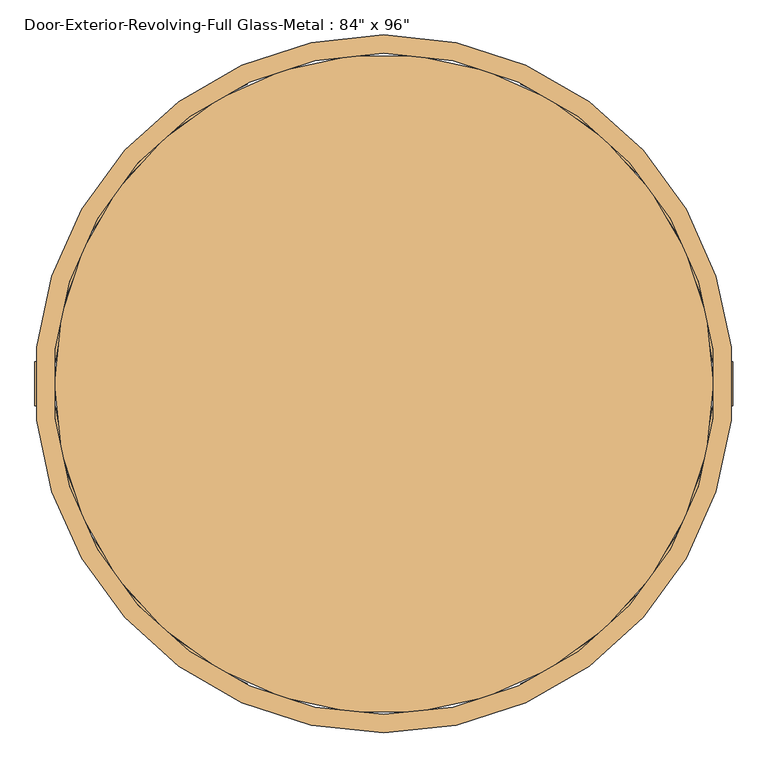
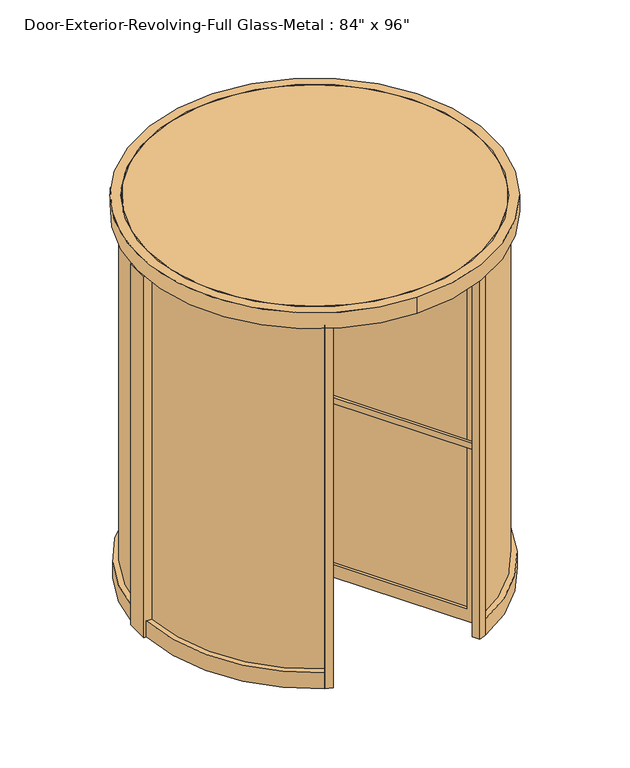
"""IFC4 building model written with IfcOpenShell, lengths in millimetres: door geometry."""

import ifcopenshell
import ifcopenshell.guid

model = None  # the IFC model being written
_history = None  # IfcOwnerHistory: only IFC2X3 demands one
_inside = {}  # id of a spatial element -> (the spatial element, [elements in it])
_under = {}  # id of a project, library or spatial element -> (it, [spatial elements below it])
_declared = {}  # id of a project -> (the project, [libraries it declares])
_typed = {}  # id of a type object -> (the type object, [elements of that type])
_made_of = {}  # id of a material, layer set ... -> (it, [elements and type objects made of it])


def new_model(schema):
    """Start an empty IFC model of exactly this schema.

    Asked for "IFC4X3", IfcOpenShell would pick the latest addendum, in which some entities
    have other attributes; the version numbers below select the first issue.
    IFC2X3 requires an IfcOwnerHistory on every rooted entity: one is made here for all.
    """
    global model, _history
    if schema == "IFC4X3":
        model = ifcopenshell.file(schema_version=(4, 3, 0, 0))
    else:
        model = ifcopenshell.file(schema=schema)
    _inside.clear()
    _under.clear()
    _declared.clear()
    _typed.clear()
    _made_of.clear()
    _history = None
    if model.schema == "IFC2X3":
        org = make("IfcOrganization", Name="unknown")
        user = make(
            "IfcPersonAndOrganization",
            ThePerson=make("IfcPerson", FamilyName="unknown"),
            TheOrganization=org,
        )
        app = make(
            "IfcApplication",
            ApplicationDeveloper=org,
            Version="unknown",
            ApplicationFullName="unknown",
            ApplicationIdentifier="unknown",
        )
        _history = make(
            "IfcOwnerHistory",
            OwningUser=user,
            OwningApplication=app,
            ChangeAction="ADDED",
            CreationDate=0,
        )
    return model


def make(cls, **values):
    """One entity of the class cls with the attributes given. An attribute that is None is left unset."""
    return model.create_entity(
        cls, **{name: value for name, value in values.items() if value is not None}
    )


def rooted(cls, **values):
    """An entity with a GlobalId (a new one), such as an element, a storey or a relation."""
    return make(cls, GlobalId=ifcopenshell.guid.new(), OwnerHistory=_history, **values)


def si_unit(unit_type, name, prefix=None):
    """IfcSIUnit, for example si_unit("LENGTHUNIT", "METRE", prefix="MILLI")."""
    return make("IfcSIUnit", UnitType=unit_type, Prefix=prefix, Name=name)


def assignment(units):
    """IfcUnitAssignment: the units of a project."""
    return None if units is None else make("IfcUnitAssignment", Units=units)


def point(xyz):
    """IfcCartesianPoint."""
    return None if xyz is None else make("IfcCartesianPoint", Coordinates=xyz)


def direction(xyz):
    """IfcDirection."""
    return None if xyz is None else make("IfcDirection", DirectionRatios=xyz)


def frame(location, z_axis=None, x_axis=None):
    """IfcAxis2Placement3D, a coordinate frame: its origin and axes. An axis left out is left unset."""
    return make(
        "IfcAxis2Placement3D",
        Location=point(location),
        Axis=direction(z_axis),
        RefDirection=direction(x_axis),
    )


def frame_2d(location, x_axis=None):
    """IfcAxis2Placement2D, a coordinate frame in the plane: its origin and x axis."""
    return make(
        "IfcAxis2Placement2D", Location=point(location), RefDirection=direction(x_axis)
    )


def origin():
    """The frame at (0, 0, 0) with its axes left unset."""
    return frame((0.0, 0.0, 0.0))


def origin_with_axes():
    """The frame at (0, 0, 0) with the z axis (0, 0, 1) and the x axis (1, 0, 0) written out."""
    return frame((0.0, 0.0, 0.0), z_axis=(0.0, 0.0, 1.0), x_axis=(1.0, 0.0, 0.0))


def origin_2d():
    """The frame at (0, 0) in the plane with its x axis left unset."""
    return frame_2d((0.0, 0.0))


def place(relative_to, where):
    """IfcLocalPlacement: puts the frame where relative to a parent placement (None: the world)."""
    return make(
        "IfcLocalPlacement", PlacementRelTo=relative_to, RelativePlacement=where
    )


def context(
    kind, dimensions, precision=None, world=None, true_north=None, identifier=None
):
    """IfcGeometricRepresentationContext, for example the 3D "Model" context."""
    return make(
        "IfcGeometricRepresentationContext",
        ContextIdentifier=identifier,
        ContextType=kind,
        CoordinateSpaceDimension=dimensions,
        Precision=precision,
        WorldCoordinateSystem=world,
        TrueNorth=true_north,
    )


def project(units=None, contexts=None):
    """IfcProject with its units and contexts."""
    return rooted(
        "IfcProject",
        Name="project",
        RepresentationContexts=contexts,
        UnitsInContext=assignment(units),
    )


def spatial(cls, under=None, at=None, **own):
    """A site, building, storey or space (cls), placed at a placement, below another one or the project."""
    s = rooted(cls, ObjectPlacement=at, **own)
    if under is not None:
        _under.setdefault(under.id(), (under, []))[1].append(s)
    return s


def polyline(points):
    """IfcPolyline through the points."""
    return make("IfcPolyline", Points=[point(p) for p in points])


def circle_curve(where, radius):
    """IfcCircle in the frame where."""
    return make("IfcCircle", Position=where, Radius=radius)


def trimmed(basis, trim1, trim2, sense, master):
    """IfcTrimmedCurve: the piece of a basis curve between two trims."""
    return make(
        "IfcTrimmedCurve",
        BasisCurve=basis,
        Trim1=trim1,
        Trim2=trim2,
        SenseAgreement=sense,
        MasterRepresentation=master,
    )


def segment(curve, same_sense, transition):
    """IfcCompositeCurveSegment."""
    return make(
        "IfcCompositeCurveSegment",
        Transition=transition,
        SameSense=same_sense,
        ParentCurve=curve,
    )


def composite_curve(segments, self_intersect=None):
    """IfcCompositeCurve: segments joined end to end."""
    return make("IfcCompositeCurve", Segments=segments, SelfIntersect=self_intersect)


def outline(outer, holes=None, kind="AREA"):
    """IfcArbitraryClosedProfileDef: a profile drawn as a closed curve; with holes, ...WithVoids."""
    if holes is None:
        return make("IfcArbitraryClosedProfileDef", ProfileType=kind, OuterCurve=outer)
    return make(
        "IfcArbitraryProfileDefWithVoids",
        ProfileType=kind,
        OuterCurve=outer,
        InnerCurves=holes,
    )


def extrude(swept, where, along, depth):
    """IfcExtrudedAreaSolid: the profile swept, set in the frame where, extruded along a direction by depth."""
    return make(
        "IfcExtrudedAreaSolid",
        SweptArea=swept,
        Position=where,
        ExtrudedDirection=direction(along),
        Depth=depth,
    )


def shape(context_of_items, identifier, shape_type, items):
    """IfcShapeRepresentation: the items that make up one representation, for example the "Body"."""
    return make(
        "IfcShapeRepresentation",
        ContextOfItems=context_of_items,
        RepresentationIdentifier=identifier,
        RepresentationType=shape_type,
        Items=items,
    )


def source(mapping_origin, context_of_items, identifier, shape_type, items):
    """IfcRepresentationMap: a shape defined once, which mapped items show again and again."""
    return make(
        "IfcRepresentationMap",
        MappingOrigin=mapping_origin,
        MappedRepresentation=shape(context_of_items, identifier, shape_type, items),
    )


def transform(
    local_origin,
    x_axis=None,
    y_axis=None,
    z_axis=None,
    scale=None,
    scale2=None,
    scale3=None,
    uniform=True,
):
    """IfcCartesianTransformationOperator3D, or its non-uniform kind. x_axis, y_axis, z_axis: its Axis1, 2, 3."""
    if uniform:
        return make(
            "IfcCartesianTransformationOperator3D",
            Axis1=direction(x_axis),
            Axis2=direction(y_axis),
            LocalOrigin=point(local_origin),
            Scale=scale,
            Axis3=direction(z_axis),
        )
    return make(
        "IfcCartesianTransformationOperator3DnonUniform",
        Axis1=direction(x_axis),
        Axis2=direction(y_axis),
        LocalOrigin=point(local_origin),
        Scale=scale,
        Axis3=direction(z_axis),
        Scale2=scale2,
        Scale3=scale3,
    )


def mapped(mapping_source, mapping_target):
    """IfcMappedItem: shows the shape of a source again, moved by a transform."""
    return make(
        "IfcMappedItem", MappingSource=mapping_source, MappingTarget=mapping_target
    )


def made_of(thing, what):
    """Note that an element or type object is made of a material, layer set ...; save() writes the relation."""
    if what is not None:
        _made_of.setdefault(what.id(), (what, []))[1].append(thing)
    return thing


def element(
    cls,
    number,
    at=None,
    inside=None,
    cuts=None,
    type_object=None,
    material=None,
    context=None,
    identifier="Body",
    shape_type=None,
    held_by="IfcProductDefinitionShape",
    body=None,
    shapes=None,
    **own,
):
    """One element of the class cls, such as IfcWall. Its Tag is "e" and its number.

    at: its placement. inside: the storey or other place that contains it. cuts: it is an
    opening in that element (IfcRelVoidsElement). A single representation is given by context,
    identifier, shape_type and body (its items); several are given by shapes. held_by: the class
    of the entity that holds the representations. save() writes the other relations.
    """
    e = rooted(cls, Tag="e%d" % number, ObjectPlacement=at, **own)
    if body is not None:
        shapes = [shape(context, identifier, shape_type, body)]
    if shapes is not None:
        e.Representation = make(held_by, Representations=shapes)
    if inside is not None:
        _inside.setdefault(inside.id(), (inside, []))[1].append(e)
    if cuts is not None:
        rooted(
            "IfcRelVoidsElement", RelatingBuildingElement=cuts, RelatedOpeningElement=e
        )
    if type_object is not None:
        _typed.setdefault(type_object.id(), (type_object, []))[1].append(e)
    return made_of(e, material)


def aggregate(whole, parts):
    """IfcRelAggregates: a whole, such as a stair, and the parts it consists of."""
    return rooted("IfcRelAggregates", RelatingObject=whole, RelatedObjects=parts)


def save(model, path):
    """Write the relations noted so far, then the file.

    IfcRelAggregates (storeys below a building ...), IfcRelContainedInSpatialStructure (elements
    in a storey), IfcRelDefinesByType, IfcRelAssociatesMaterial and IfcRelDeclares: one each for
    every whole, place, type object, material and project.
    """
    for whole, parts in _under.values():
        aggregate(whole, parts)
    for where, things in _inside.values():
        rooted(
            "IfcRelContainedInSpatialStructure",
            RelatedElements=things,
            RelatingStructure=where,
        )
    for kind, things in _typed.values():
        rooted("IfcRelDefinesByType", RelatedObjects=things, RelatingType=kind)
    for what, things in _made_of.values():
        rooted("IfcRelAssociatesMaterial", RelatedObjects=things, RelatingMaterial=what)
    for by, libraries in _declared.values():
        rooted("IfcRelDeclares", RelatingContext=by, RelatedDefinitions=libraries)
    model.write(path)


def plane_surface(at):
    """IfcPlane: the flat surface through the origin of the frame at, square to its z axis."""
    return make("IfcPlane", Position=at)


def revolved_surface(curve, axis_point, axis_direction):
    """IfcSurfaceOfRevolution: the curve turned about the line through axis_point along axis_direction."""
    return make(
        "IfcSurfaceOfRevolution",
        SweptCurve=make("IfcArbitraryOpenProfileDef", ProfileType="CURVE", Curve=curve),
        AxisPosition=make("IfcAxis1Placement", Location=point(axis_point), Axis=direction(axis_direction)),
    )


def advanced_brep(points, edges, surfaces, faces):
    """IfcAdvancedBrep: a solid bounded by faces that lie on surfaces and meet in shared edges.

    An edge is (start, end): straight between two places in points (the first is 0);
    or (start, end, curve); or (start, end, curve, False) where it runs against its curve.
    A face is (place in surfaces, loops), or (place, loops, False) where it looks against
    its surface's normal. A loop lists edges by number (the first is 1), with a minus sign
    where the edge is run from its end to its start. The first loop is the outer one.
    """
    corners = [point(p) for p in points]
    vertices = [make("IfcVertexPoint", VertexGeometry=c) for c in corners]
    made = []
    for start, end, *more in edges:
        made.append(
            make(
                "IfcEdgeCurve",
                EdgeStart=vertices[start],
                EdgeEnd=vertices[end],
                EdgeGeometry=more[0] if more else make("IfcPolyline", Points=[corners[start], corners[end]]),
                SameSense=more[1] if len(more) > 1 else True,
            )
        )
    hull = []
    for where, loops, *sense in faces:
        bounds = []
        for j, loop in enumerate(loops):
            ring = [make("IfcOrientedEdge", EdgeElement=made[abs(k) - 1], Orientation=k > 0) for k in loop]
            bounds.append(
                make(
                    "IfcFaceOuterBound" if j == 0 else "IfcFaceBound",
                    Bound=make("IfcEdgeLoop", EdgeList=ring),
                    Orientation=True,
                )
            )
        hull.append(make("IfcAdvancedFace", Bounds=bounds, FaceSurface=surfaces[where], SameSense=sense[0] if sense else True))
    return make("IfcAdvancedBrep", Outer=make("IfcClosedShell", CfsFaces=hull))


def door_2695eedf(model_context):
    return source(origin(), model_context, "Body", "SolidModel", [
        advanced_brep(
        [(481.9772161, -872.9090263, 25.4), (481.9772161, -872.9090263, 2282.825), (26.9196881, -84.7262674, 2282.825), (26.9196881, -84.7262674, 25.4), (29.5397161, -89.2642891, 2216.15), (448.6397161, -815.1667825, 2216.15), (448.6397161, -815.1667825, 106.3625), (29.5397161, -89.2642891, 106.3625), (514.9727839, -853.8590263, 2282.825), (514.9727839, -853.8590263, 25.4), (59.9152559, -65.6762674, 25.4), (59.9152559, -65.6762674, 2282.825), (62.5352839, -70.2142891, 2216.15), (62.5352839, -70.2142891, 106.3625), (481.6352839, -796.1167825, 106.3625), (481.6352839, -796.1167825, 2216.15), (44.45, -76.9896584, 2282.825), (44.45, -76.9896584, 25.4)],
        [
            (0, 1),
            (1, 2),
            (2, 3),
            (3, 0),
            (4, 5),
            (5, 6),
            (6, 7),
            (7, 4),
            (8, 9),
            (9, 10),
            (10, 11),
            (11, 8),
            (12, 13),
            (13, 14),
            (14, 15),
            (15, 12),
            (1, 8),
            (11, 16, circle_curve(frame((0.0, 0.0, 2282.825), z_axis=(0.0, 0.0, -1.0), x_axis=(0.4999999999999996, -0.8660254037844389, 0.0)), 88.9)),
            (16, 2, circle_curve(frame((0.0, 0.0, 2282.825), z_axis=(0.0, 0.0, -1.0), x_axis=(0.4999999999999996, -0.8660254037844389, 0.0)), 88.9)),
            (0, 9),
            (3, 17, circle_curve(frame((0.0, 0.0, 25.4), z_axis=(0.0, 0.0, 1.0), x_axis=(0.4999999999999996, -0.8660254037844389, 0.0)), 88.9)),
            (17, 10, circle_curve(frame((0.0, 0.0, 25.4), z_axis=(0.0, 0.0, 1.0), x_axis=(0.4999999999999996, -0.8660254037844389, 0.0)), 88.9)),
            (7, 13),
            (12, 4),
            (6, 14),
            (5, 15),
            (16, 17),
        ],
        [
            plane_surface(frame((-3.7977839, -31.5220453, 2282.825), z_axis=(-0.8660254037844389, -0.4999999999999996, 0.0), x_axis=(0.0, 0.0, -1.0))),
            plane_surface(frame((29.1977839, -12.4720453, 2282.825), z_axis=(0.8660254037844389, 0.4999999999999996, 0.0), x_axis=(0.0, 0.0, 1.0))),
            plane_surface(frame((481.9772161, -872.9090263, 2282.825), z_axis=(0.0, 0.0, 1.0), x_axis=(0.8660254037844384, 0.5000000000000004, 0.0))),
            plane_surface(frame((481.9772161, -872.9090263, 25.4), z_axis=(0.5000000000000004, -0.8660254037844384, 0.0), x_axis=(0.8660254037844384, 0.5000000000000004, 0.0))),
            plane_surface(frame((-3.7977839, -31.5220453, 25.4), z_axis=(0.0, 0.0, -1.0), x_axis=(0.8660254037844389, 0.49999999999999956, 0.0))),
            plane_surface(frame((29.5397161, -89.2642891, 106.3625), z_axis=(0.4999999999999998, -0.8660254037844388, 0.0), x_axis=(0.8660254037844388, 0.4999999999999998, 0.0))),
            plane_surface(frame((448.6397161, -815.1667825, 106.3625), z_axis=(0.0, 0.0, 1.0), x_axis=(0.8660254037844384, 0.5000000000000004, 0.0))),
            plane_surface(frame((448.6397161, -815.1667825, 2216.15), z_axis=(-0.5000000000000004, 0.8660254037844384, 0.0), x_axis=(0.8660254037844384, 0.5000000000000004, 0.0))),
            plane_surface(frame((29.5397161, -89.2642891, 2216.15), z_axis=(0.0, 0.0, -1.0), x_axis=(0.8660254037844389, 0.49999999999999967, 0.0))),
            revolved_surface(polyline([(44.44999999999997, -76.98965839643662, 2282.825), (44.44999999999997, -76.98965839643662, 25.399999999999977)]), (0.0, 0.0, -344.4385455), (0.0, 0.0, 1.0)),
        ],
        [
            (0, [[1, 2, 3, 4], [5, 6, 7, 8]]),
            (1, [[9, 10, 11, 12], [13, 14, 15, 16]]),
            (2, [[17, -12, 18, 19, -2]]),
            (3, [[-1, 20, -9, -17]]),
            (4, [[-20, -4, 21, 22, -10]]),
            (5, [[-8, 23, -13, 24]]),
            (6, [[-7, 25, -14, -23]]),
            (7, [[-6, 26, -15, -25]]),
            (8, [[-5, -24, -16, -26]]),
            (9, [[27, -21, -3, -19]]),
            (9, [[-27, -18, -11, -22]]),
        ],
    ),
        advanced_brep(
        [(-996.95, -19.05, 2282.825), (-996.95, -19.05, 25.4), (-86.834944, -19.05, 25.4), (-86.834944, -19.05, 2282.825), (-92.075, -19.05, 2216.15), (-92.075, -19.05, 106.3625), (-930.275, -19.05, 106.3625), (-930.275, -19.05, 2216.15), (-996.95, 19.05, 25.4), (-996.95, 19.05, 2282.825), (-86.834944, 19.05, 2282.825), (-86.834944, 19.05, 25.4), (-92.075, 19.05, 2216.15), (-930.275, 19.05, 2216.15), (-930.275, 19.05, 106.3625), (-92.075, 19.05, 106.3625)],
        [
            (0, 1),
            (1, 2),
            (2, 3),
            (3, 0),
            (4, 5),
            (5, 6),
            (6, 7),
            (7, 4),
            (8, 9),
            (9, 10),
            (10, 11),
            (11, 8),
            (12, 13),
            (13, 14),
            (14, 15),
            (15, 12),
            (9, 0),
            (3, 10, circle_curve(frame((0.0, 0.0, 2282.825), z_axis=(0.0, 0.0, -1.0), x_axis=(0.4999999999999996, -0.8660254037844389, 0.0)), 88.9)),
            (8, 1),
            (11, 2, circle_curve(frame((0.0, 0.0, 25.4), z_axis=(0.0, 0.0, 1.0), x_axis=(0.4999999999999996, -0.8660254037844389, 0.0)), 88.9)),
            (4, 12),
            (15, 5),
            (14, 6),
            (13, 7),
        ],
        [
            plane_surface(frame((-996.95, -19.05, 2282.825), z_axis=(0.0, -1.0, 0.0), x_axis=(-1.0, 0.0, 0.0))),
            plane_surface(frame((-996.95, 19.05, 2282.825), z_axis=(0.0, 1.0, 0.0), x_axis=(1.0, 0.0, 0.0))),
            plane_surface(frame((-25.4, -19.05, 2282.825), z_axis=(0.0, 0.0, 1.0), x_axis=(0.0, 1.0, 0.0))),
            plane_surface(frame((-996.95, -19.05, 2282.825), z_axis=(-1.0, 0.0, 0.0), x_axis=(0.0, 1.0, 0.0))),
            plane_surface(frame((-996.95, -19.05, 25.4), z_axis=(0.0, 0.0, -1.0), x_axis=(0.0, 1.0, 0.0))),
            plane_surface(frame((-92.075, -19.05, 2216.15), z_axis=(-1.0, 0.0, 0.0), x_axis=(0.0, 1.0, 0.0))),
            plane_surface(frame((-92.075, -19.05, 106.3625), z_axis=(0.0, 0.0, 1.0), x_axis=(0.0, 1.0, 0.0))),
            plane_surface(frame((-930.275, -19.05, 106.3625), z_axis=(1.0, 0.0, 0.0), x_axis=(0.0, 1.0, 0.0))),
            plane_surface(frame((-930.275, -19.05, 2216.15), z_axis=(0.0, 0.0, -1.0), x_axis=(0.0, 1.0, 0.0))),
            revolved_surface(polyline([(44.44999999999997, -76.98965839643662, 2282.825), (44.44999999999997, -76.98965839643662, 25.399999999999977)]), (0.0, 0.0, -344.4385455), (0.0, 0.0, 1.0)),
        ],
        [
            (0, [[1, 2, 3, 4], [5, 6, 7, 8]]),
            (1, [[9, 10, 11, 12], [13, 14, 15, 16]]),
            (2, [[17, -4, 18, -10]]),
            (3, [[-1, -17, -9, 19]]),
            (4, [[-19, -12, 20, -2]]),
            (5, [[-5, 21, -16, 22]]),
            (6, [[-6, -22, -15, 23]]),
            (7, [[-7, -23, -14, 24]]),
            (8, [[-8, -24, -13, -21]]),
            (9, [[-3, -20, -11, -18]]),
        ],
    ),
        advanced_brep(
        [(514.9727839, 853.8590263, 25.4), (514.9727839, 853.8590263, 2282.825), (59.9152559, 65.6762674, 2282.825), (59.9152559, 65.6762674, 25.4), (62.5352839, 70.2142891, 2216.15), (481.6352839, 796.1167825, 2216.15), (481.6352839, 796.1167825, 106.3625), (62.5352839, 70.2142891, 106.3625), (481.9772161, 872.9090263, 2282.825), (481.9772161, 872.9090263, 25.4), (26.9196881, 84.7262674, 25.4), (26.9196881, 84.7262674, 2282.825), (29.5397161, 89.2642891, 2216.15), (29.5397161, 89.2642891, 106.3625), (448.6397161, 815.1667825, 106.3625), (448.6397161, 815.1667825, 2216.15)],
        [
            (0, 1),
            (1, 2),
            (2, 3),
            (3, 0),
            (4, 5),
            (5, 6),
            (6, 7),
            (7, 4),
            (8, 9),
            (9, 10),
            (10, 11),
            (11, 8),
            (12, 13),
            (13, 14),
            (14, 15),
            (15, 12),
            (1, 8),
            (11, 2, circle_curve(frame((0.0, 0.0, 2282.825), z_axis=(0.0, 0.0, -1.0), x_axis=(0.4999999999999996, -0.8660254037844389, 0.0)), 88.9)),
            (0, 9),
            (3, 10, circle_curve(frame((0.0, 0.0, 25.4), z_axis=(0.0, 0.0, 1.0), x_axis=(0.4999999999999996, -0.8660254037844389, 0.0)), 88.9)),
            (7, 13),
            (12, 4),
            (6, 14),
            (5, 15),
        ],
        [
            plane_surface(frame((29.1977839, 12.4720453, 2282.825), z_axis=(0.866025403784439, -0.4999999999999995, 0.0), x_axis=(0.0, 0.0, -1.0))),
            plane_surface(frame((-3.7977839, 31.5220453, 2282.825), z_axis=(-0.866025403784439, 0.4999999999999995, 0.0), x_axis=(0.0, 0.0, 1.0))),
            plane_surface(frame((514.9727839, 853.8590263, 2282.825), z_axis=(0.0, 0.0, 1.0), x_axis=(-0.8660254037844384, 0.5000000000000004, 0.0))),
            plane_surface(frame((514.9727839, 853.8590263, 25.4), z_axis=(0.5000000000000004, 0.8660254037844384, 0.0), x_axis=(-0.8660254037844384, 0.5000000000000004, 0.0))),
            plane_surface(frame((29.1977839, 12.4720453, 25.4), z_axis=(0.0, 0.0, -1.0), x_axis=(-0.866025403784439, 0.49999999999999944, 0.0))),
            plane_surface(frame((62.5352839, 70.2142891, 106.3625), z_axis=(0.49999999999999956, 0.8660254037844389, 0.0), x_axis=(-0.8660254037844389, 0.49999999999999956, 0.0))),
            plane_surface(frame((481.6352839, 796.1167825, 106.3625), z_axis=(0.0, 0.0, 1.0), x_axis=(-0.8660254037844384, 0.5000000000000004, 0.0))),
            plane_surface(frame((481.6352839, 796.1167825, 2216.15), z_axis=(-0.5000000000000004, -0.8660254037844384, 0.0), x_axis=(-0.8660254037844384, 0.5000000000000004, 0.0))),
            plane_surface(frame((62.5352839, 70.2142891, 2216.15), z_axis=(0.0, 0.0, -1.0), x_axis=(-0.866025403784439, 0.49999999999999944, 0.0))),
            revolved_surface(polyline([(44.44999999999997, -76.98965839643662, 2282.825), (44.44999999999997, -76.98965839643662, 25.399999999999977)]), (0.0, 0.0, -344.4385455), (0.0, 0.0, 1.0)),
        ],
        [
            (0, [[1, 2, 3, 4], [5, 6, 7, 8]]),
            (1, [[9, 10, 11, 12], [13, 14, 15, 16]]),
            (2, [[17, -12, 18, -2]]),
            (3, [[-1, 19, -9, -17]]),
            (4, [[-19, -4, 20, -10]]),
            (5, [[-8, 21, -13, 22]]),
            (6, [[-7, 23, -14, -21]]),
            (7, [[-6, 24, -15, -23]]),
            (8, [[-5, -22, -16, -24]]),
            (9, [[-3, -18, -11, -20]]),
        ],
    ),
        extrude(outline(composite_curve([segment(polyline([(-463.3921907, 900.6009984), (-485.7275667, 942.9715583)]), True, "CONTINUOUS"), segment(trimmed(circle_curve(origin_2d(), 1060.7198635), [point((-485.7275667, 942.9715583))], [point((-443.2078601, 963.6874086))], False, "CARTESIAN"), True, "CONTINUOUS"), segment(polyline([(-443.2078601, 963.6874086), (-420.8795251, 921.2355323)]), True, "CONTINUOUS"), segment(trimmed(circle_curve(origin_2d(), 1012.825), [point((-420.8795251, 921.2355323))], [point((-463.3921907, 900.6009984))], True, "CARTESIAN"), True, "CONTINUOUS")], self_intersect=False)), origin_with_axes(), (0.0, 0.0, 1.0), 2308.225),
        extrude(outline(composite_curve([segment(polyline([(485.8334006, 943.1723269), (463.3921907, 900.6009984)]), True, "CONTINUOUS"), segment(trimmed(circle_curve(origin_2d(), 1012.825), [point((463.3921907, 900.6009984))], [point((420.8795251, 921.2355323))], True, "CARTESIAN"), True, "CONTINUOUS"), segment(polyline([(420.8795251, 921.2355323), (443.3136707, 963.8885416)]), True, "CONTINUOUS"), segment(trimmed(circle_curve(origin_2d(), 1060.9468089), [point((443.3136707, 963.8885416))], [point((485.8334006, 943.1723269))], False, "CARTESIAN"), True, "CONTINUOUS")], self_intersect=False)), origin_with_axes(), (0.0, 0.0, 1.0), 2308.225),
        extrude(outline(composite_curve([segment(trimmed(circle_curve(origin_2d(), 1012.825), [point((-463.3921907, -900.6009984))], [point((-420.8795251, -921.2355323))], True, "CARTESIAN"), True, "CONTINUOUS"), segment(polyline([(-420.8795251, -921.2355323), (-443.2078601, -959.6749591)]), True, "CONTINUOUS"), segment(trimmed(circle_curve(frame_2d((0.0, 231.0126656)), 1270.4999909), [point((-443.2078601, -959.6749591))], [point((-485.7275667, -942.9715583))], False, "CARTESIAN"), True, "CONTINUOUS"), segment(polyline([(-485.7275667, -942.9715583), (-463.3921907, -900.6009984)]), True, "CONTINUOUS")], self_intersect=False)), origin_with_axes(), (0.0, 0.0, 1.0), 2308.225),
        extrude(outline(composite_curve([segment(trimmed(circle_curve(frame_2d((0.0, 231.0127852)), 1270.5001015), [point((485.7275667, -942.9715583))], [point((443.2078689, -959.6749542))], False, "CARTESIAN"), True, "CONTINUOUS"), segment(polyline([(443.2078689, -959.6749542), (420.8795251, -921.2355323)]), True, "CONTINUOUS"), segment(trimmed(circle_curve(origin_2d(), 1012.825), [point((420.8795251, -921.2355323))], [point((463.3921907, -900.6009984))], True, "CARTESIAN"), True, "CONTINUOUS"), segment(polyline([(463.3921907, -900.6009984), (485.7275667, -942.9715583)]), True, "CONTINUOUS")], self_intersect=False)), origin_with_axes(), (0.0, 0.0, 1.0), 2308.225),
        extrude(outline(composite_curve([segment(polyline([(-1018.5303379, 67.46875), (-1024.8907518, 67.46875)]), True, "CONTINUOUS"), segment(trimmed(circle_curve(origin_2d(), 1027.1090913), [point((-1024.8907518, 67.46875))], [point((-470.5714922, 912.9707312))], False, "CARTESIAN"), True, "CONTINUOUS"), segment(polyline([(-470.5714922, 912.9707312), (-467.3807004, 907.4752681)]), True, "CONTINUOUS"), segment(trimmed(circle_curve(origin_2d(), 1020.7625), [point((-467.3807004, 907.4752681))], [point((-1018.5303379, 67.46875))], True, "CARTESIAN"), True, "CONTINUOUS")], self_intersect=False)), frame((0.0, 0.0, 101.6), z_axis=(0.0, 0.0, 1.0), x_axis=(1.0, 0.0, 0.0)), (0.0, 0.0, 1.0), 2206.625),
        extrude(outline(composite_curve([segment(trimmed(circle_curve(origin_2d(), 1020.7625), [point((1018.5303379, 67.46875))], [point((467.3807004, 907.4752681))], True, "CARTESIAN"), True, "CONTINUOUS"), segment(polyline([(467.3807004, 907.4752681), (470.5714922, 912.9707312)]), True, "CONTINUOUS"), segment(trimmed(circle_curve(origin_2d(), 1027.1090913), [point((470.5714922, 912.9707312))], [point((1024.8907518, 67.46875))], False, "CARTESIAN"), True, "CONTINUOUS"), segment(polyline([(1024.8907518, 67.46875), (1018.5303379, 67.46875)]), True, "CONTINUOUS")], self_intersect=False)), frame((0.0, 0.0, 101.6), z_axis=(0.0, 0.0, 1.0), x_axis=(1.0, 0.0, 0.0)), (0.0, 0.0, 1.0), 2206.625),
        extrude(outline(composite_curve([segment(trimmed(circle_curve(origin_2d(), 1020.7625), [point((-1018.5303379, -67.46875))], [point((-467.3807004, -907.4752681))], True, "CARTESIAN"), True, "CONTINUOUS"), segment(polyline([(-467.3807004, -907.4752681), (-470.5714922, -912.9707312)]), True, "CONTINUOUS"), segment(trimmed(circle_curve(origin_2d(), 1027.1090913), [point((-470.5714922, -912.9707312))], [point((-1024.8907518, -67.46875))], False, "CARTESIAN"), True, "CONTINUOUS"), segment(polyline([(-1024.8907518, -67.46875), (-1018.5303379, -67.46875)]), True, "CONTINUOUS")], self_intersect=False)), frame((0.0, 0.0, 101.6), z_axis=(0.0, 0.0, 1.0), x_axis=(1.0, 0.0, 0.0)), (0.0, 0.0, 1.0), 2206.625),
        extrude(outline(composite_curve([segment(polyline([(1018.5303379, -67.46875), (1024.8907518, -67.46875)]), True, "CONTINUOUS"), segment(trimmed(circle_curve(origin_2d(), 1027.1090913), [point((1024.8907518, -67.46875))], [point((470.5714922, -912.9707312))], False, "CARTESIAN"), True, "CONTINUOUS"), segment(polyline([(470.5714922, -912.9707312), (467.3807004, -907.4752681)]), True, "CONTINUOUS"), segment(trimmed(circle_curve(origin_2d(), 1020.7625), [point((467.3807004, -907.4752681))], [point((1018.5303379, -67.46875))], True, "CARTESIAN"), True, "CONTINUOUS")], self_intersect=False)), frame((0.0, 0.0, 101.6), z_axis=(0.0, 0.0, 1.0), x_axis=(1.0, 0.0, 0.0)), (0.0, 0.0, 1.0), 2206.625),
        extrude(outline(composite_curve([segment(trimmed(circle_curve(origin_2d(), 1073.15), [point((0.0, -1073.15))], [point((0.0, 1073.15))], False, "CARTESIAN"), True, "CONTINUOUS"), segment(trimmed(circle_curve(origin_2d(), 1073.15), [point((0.0, 1073.15))], [point((0.0, -1073.15))], False, "CARTESIAN"), True, "CONTINUOUS")], self_intersect=False), holes=[composite_curve([segment(trimmed(circle_curve(origin_2d(), 1016.0), [point((0.0, 1016.0))], [point((0.0, -1016.0))], True, "CARTESIAN"), True, "CONTINUOUS"), segment(trimmed(circle_curve(origin_2d(), 1016.0), [point((0.0, -1016.0))], [point((0.0, 1016.0))], True, "CARTESIAN"), True, "CONTINUOUS")], self_intersect=False)]), frame((0.0, 0.0, 2308.225), z_axis=(0.0, 0.0, 1.0), x_axis=(1.0, 0.0, 0.0)), (0.0, 0.0, 1.0), 101.6),
        extrude(outline(composite_curve([segment(trimmed(circle_curve(origin_2d(), 1012.825), [point((-1012.825, 0.0))], [point((1012.825, 0.0))], False, "CARTESIAN"), True, "CONTINUOUS"), segment(trimmed(circle_curve(origin_2d(), 1012.825), [point((1012.825, 0.0))], [point((-1012.825, 0.0))], False, "CARTESIAN"), True, "CONTINUOUS")], self_intersect=False)), frame((0.0, 0.0, 2308.225), z_axis=(0.0, 0.0, 1.0), x_axis=(1.0, 0.0, 0.0)), (0.0, 0.0, 1.0), 101.6),
        extrude(outline(composite_curve([segment(trimmed(circle_curve(origin_2d(), 88.9), [point((-88.9, 0.0))], [point((88.9, 0.0))], False, "CARTESIAN"), True, "CONTINUOUS"), segment(trimmed(circle_curve(origin_2d(), 88.9), [point((88.9, 0.0))], [point((-88.9, 0.0))], False, "CARTESIAN"), True, "CONTINUOUS")], self_intersect=False)), origin_with_axes(), (0.0, 0.0, 1.0), 2308.225),
        extrude(outline(composite_curve([segment(polyline([(-463.3921907, -900.6009984), (-485.7275667, -942.9715583)]), True, "CONTINUOUS"), segment(trimmed(circle_curve(origin_2d(), 1060.7198635), [point((-485.7275667, -942.9715583))], [point((-1058.571961, -67.46875))], False, "CARTESIAN"), True, "CONTINUOUS"), segment(polyline([(-1058.571961, -67.46875), (-1010.5753057, -67.46875)]), True, "CONTINUOUS"), segment(trimmed(circle_curve(origin_2d(), 1012.825), [point((-1010.5753057, -67.46875))], [point((-463.3921907, -900.6009984))], True, "CARTESIAN"), True, "CONTINUOUS")], self_intersect=False)), origin_with_axes(), (0.0, 0.0, 1.0), 101.6),
        extrude(outline(composite_curve([segment(polyline([(485.7275667, -942.9715583), (463.3921907, -900.6009984)]), True, "CONTINUOUS"), segment(trimmed(circle_curve(origin_2d(), 1012.825), [point((463.3921907, -900.6009984))], [point((1010.5753057, -67.46875))], True, "CARTESIAN"), True, "CONTINUOUS"), segment(polyline([(1010.5753057, -67.46875), (1058.571961, -67.46875)]), True, "CONTINUOUS"), segment(trimmed(circle_curve(origin_2d(), 1060.7198635), [point((1058.571961, -67.46875))], [point((485.7275667, -942.9715583))], False, "CARTESIAN"), True, "CONTINUOUS")], self_intersect=False)), origin_with_axes(), (0.0, 0.0, 1.0), 101.6),
        extrude(outline(composite_curve([segment(polyline([(1058.571961, 67.46875), (1010.5753057, 67.46875)]), True, "CONTINUOUS"), segment(trimmed(circle_curve(origin_2d(), 1012.825), [point((1010.5753057, 67.46875))], [point((463.3921907, 900.6009984))], True, "CARTESIAN"), True, "CONTINUOUS"), segment(polyline([(463.3921907, 900.6009984), (485.7275667, 942.9715583)]), True, "CONTINUOUS"), segment(trimmed(circle_curve(origin_2d(), 1060.7198635), [point((485.7275667, 942.9715583))], [point((1058.571961, 67.46875))], False, "CARTESIAN"), True, "CONTINUOUS")], self_intersect=False)), origin_with_axes(), (0.0, 0.0, 1.0), 101.6),
        extrude(outline(composite_curve([segment(polyline([(-485.7275667, 942.9715583), (-463.3921907, 900.6009984)]), True, "CONTINUOUS"), segment(trimmed(circle_curve(origin_2d(), 1012.825), [point((-463.3921907, 900.6009984))], [point((-1010.5753057, 67.46875))], True, "CARTESIAN"), True, "CONTINUOUS"), segment(polyline([(-1010.5753057, 67.46875), (-1058.571961, 67.46875)]), True, "CONTINUOUS"), segment(trimmed(circle_curve(origin_2d(), 1060.7198635), [point((-1058.571961, 67.46875))], [point((-485.7275667, 942.9715583))], False, "CARTESIAN"), True, "CONTINUOUS")], self_intersect=False)), origin_with_axes(), (0.0, 0.0, 1.0), 101.6),
        extrude(outline(polyline([(-1016.0, 67.46875), (-1016.0, -67.46875), (-1073.15, -67.46875), (-1073.15, 67.46875), (-1016.0, 67.46875)])), origin_with_axes(), (0.0, 0.0, 1.0), 2308.225),
        extrude(outline(polyline([(1073.15, 67.46875), (1073.15, -67.46875), (1016.0, -67.46875), (1016.0, 67.46875), (1073.15, 67.46875)])), origin_with_axes(), (0.0, 0.0, 1.0), 2308.225),
        extrude(outline(polyline([(462.3878693, -807.2292825), (43.2878693, -81.3267891), (48.7871307, -78.1517891), (467.8871307, -804.0542825), (462.3878693, -807.2292825)])), frame((0.0, 0.0, 106.3625), z_axis=(0.0, 0.0, 1.0), x_axis=(1.0, 0.0, 0.0)), (0.0, 0.0, 1.0), 2109.7875),
        extrude(outline(polyline([(467.8871307, 804.0542825), (48.7871307, 78.1517891), (43.2878693, 81.3267891), (462.3878693, 807.2292825), (467.8871307, 804.0542825)])), frame((0.0, 0.0, 106.3625), z_axis=(0.0, 0.0, 1.0), x_axis=(1.0, 0.0, 0.0)), (0.0, 0.0, 1.0), 2109.7875),
        extrude(outline(polyline([(-92.075, -3.175), (-930.275, -3.175), (-930.275, 3.175), (-92.075, 3.175), (-92.075, -3.175)])), frame((0.0, 0.0, 106.3625), z_axis=(0.0, 0.0, 1.0), x_axis=(1.0, 0.0, 0.0)), (0.0, 0.0, 1.0), 2109.7875),
        extrude(outline(composite_curve([segment(polyline([(-996.95, 19.05), (-996.95, 38.1), (-80.3218526, 38.1)]), True, "CONTINUOUS"), segment(trimmed(circle_curve(origin_2d(), 88.9), [point((-80.3218526, 38.1))], [point((-86.834944, 19.05))], True, "CARTESIAN"), True, "CONTINUOUS"), segment(polyline([(-86.834944, 19.05), (-996.95, 19.05)]), True, "CONTINUOUS")], self_intersect=False)), frame((0.0, 0.0, 1149.35), z_axis=(0.0, 0.0, 1.0), x_axis=(1.0, 0.0, 0.0)), (0.0, 0.0, 1.0), 38.1),
        extrude(outline(composite_curve([segment(polyline([(481.9772161, -872.9090263), (465.4794321, -882.4340263), (7.1653584, -88.6107648)]), True, "CONTINUOUS"), segment(trimmed(circle_curve(origin_2d(), 88.9), [point((7.1653584, -88.6107648))], [point((26.9196881, -84.7262674))], True, "CARTESIAN"), True, "CONTINUOUS"), segment(polyline([(26.9196881, -84.7262674), (481.9772161, -872.9090263)]), True, "CONTINUOUS")], self_intersect=False)), frame((0.0, 0.0, 1149.35), z_axis=(0.0, 0.0, 1.0), x_axis=(1.0, 0.0, 0.0)), (0.0, 0.0, 1.0), 38.1),
        extrude(outline(composite_curve([segment(polyline([(514.9727839, 853.8590263), (531.4705679, 844.3340263), (73.1564942, 50.5107648)]), True, "CONTINUOUS"), segment(trimmed(circle_curve(origin_2d(), 88.9), [point((73.1564942, 50.5107648))], [point((59.9152559, 65.6762674))], True, "CARTESIAN"), True, "CONTINUOUS"), segment(polyline([(59.9152559, 65.6762674), (514.9727839, 853.8590263)]), True, "CONTINUOUS")], self_intersect=False)), frame((0.0, 0.0, 1149.35), z_axis=(0.0, 0.0, 1.0), x_axis=(1.0, 0.0, 0.0)), (0.0, 0.0, 1.0), 38.1),
    ])


if __name__ == "__main__":
    model = new_model("IFC4")
    model_context = context("Model", 3, world=origin())
    ifc_project = project(units=[si_unit("LENGTHUNIT", "METRE", prefix="MILLI")], contexts=[model_context])
    site = spatial("IfcSite", under=ifc_project)
    building = spatial("IfcBuilding", under=site)
    placement = place(None, origin())
    door_shape = door_2695eedf(model_context)
    element("IfcDoor", 1, ObjectType="Door-Exterior-Revolving-Full Glass-Metal : 84\" x 96\"", at=placement, inside=building, context=model_context, shape_type="MappedRepresentation", body=[
        mapped(door_shape, transform((0.0, 0.0, 0.0), x_axis=(1.0, 0.0, 0.0), y_axis=(0.0, 1.0, 0.0), z_axis=(0.0, 0.0, 1.0))),
    ])
    save(model, "model.ifc")

# Revit data of these elements
# Type "Door-Exterior-Revolving-Full Glass-Metal : 84\" x 96\""
#   Type Mark = "19"
#   Assembly Code = "B2030100"
#   Analytic Construction = "Metal frame, double glass door"
#   Panel Width = 3' - 2 1/4"
#   Thermal Resistance (R) = 1.3794 (h·ft²·°F)/BTU
#   Rough Width = 7' - 0 1/2"
#   Rough Height = 7' - 10 7/8"
#   Outside Diameter = 7' - 0 1/2"
#   Push Bar Height = 3' - 10"
#   Inside Radius = 3' - 3 7/8"
#   Inside Diameter = 6' - 7 3/4"
#   Heat Transfer Coefficient (U) = 0.7250 BTU/(h·ft²·°F)
#   Glazing Radius = 3' - 4 3/16"
#   Height = 7' - 10 1/2"
#   Width = 7' - 0"
#   Door Opening Width = 2' - 9 1/8"
#   Function = 1
#   Push Bar Material = Aluminum
#   Panel Material = Aluminum
#   Glazing = Glass
#   Frame Material = Aluminum
#   Visual Light Transmittance = 0
#   Solar Heat Gain Coefficient = 0
#   Wall Closure = (empty or 0)
# Element 1 (IfcDoor, "Door-Exterior-Revolving-Full Glass-Metal : 84\" x 96\"")
#   Materials on its faces: "Aluminum", "Glass"
# Materials
#   "Aluminum": class "Metal", colour RGB 247 247 247, transparency 0, Description = "Aluminum 6061", Cost = 0
#   "Glass": class "Glass", colour RGB 0 128 192, transparency 0.75, Description = "Soda Lime Glass", Cost = 0
